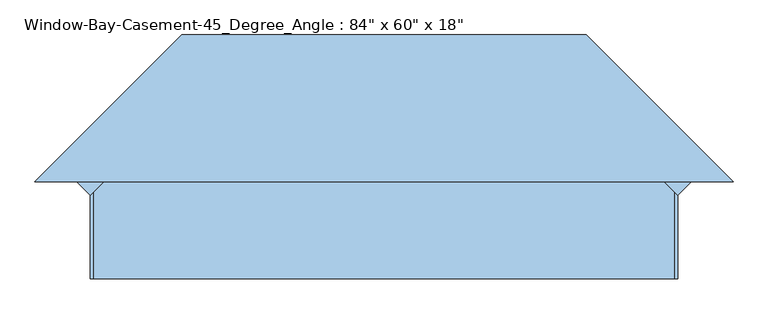
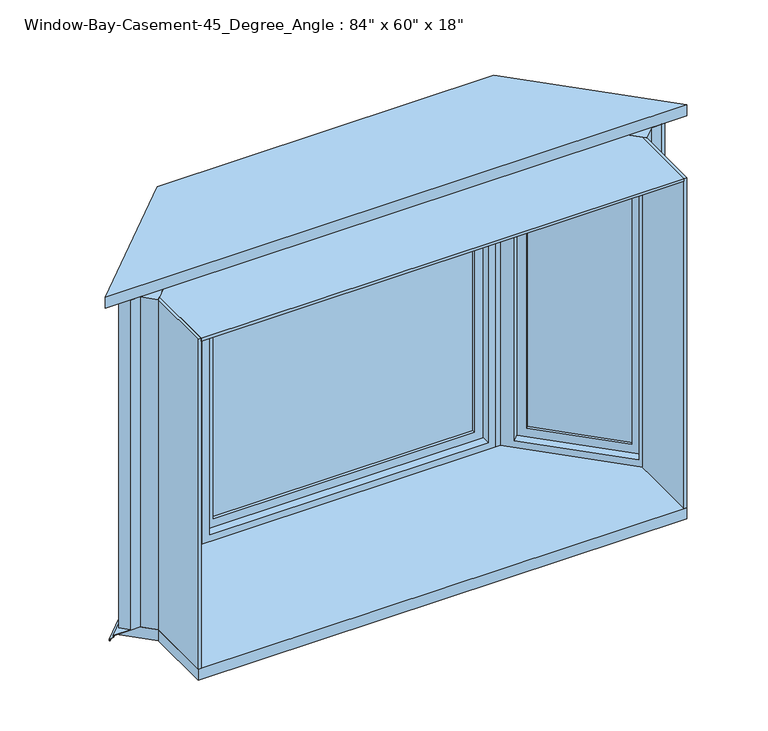
"""IFC4 building model written with IfcOpenShell, lengths in millimetres: window geometry."""

import ifcopenshell
import ifcopenshell.guid

model = None  # the IFC model being written
_history = None  # IfcOwnerHistory: only IFC2X3 demands one
_inside = {}  # id of a spatial element -> (the spatial element, [elements in it])
_under = {}  # id of a project, library or spatial element -> (it, [spatial elements below it])
_declared = {}  # id of a project -> (the project, [libraries it declares])
_typed = {}  # id of a type object -> (the type object, [elements of that type])
_made_of = {}  # id of a material, layer set ... -> (it, [elements and type objects made of it])


def new_model(schema):
    """Start an empty IFC model of exactly this schema.

    Asked for "IFC4X3", IfcOpenShell would pick the latest addendum, in which some entities
    have other attributes; the version numbers below select the first issue.
    IFC2X3 requires an IfcOwnerHistory on every rooted entity: one is made here for all.
    """
    global model, _history
    if schema == "IFC4X3":
        model = ifcopenshell.file(schema_version=(4, 3, 0, 0))
    else:
        model = ifcopenshell.file(schema=schema)
    _inside.clear()
    _under.clear()
    _declared.clear()
    _typed.clear()
    _made_of.clear()
    _history = None
    if model.schema == "IFC2X3":
        org = make("IfcOrganization", Name="unknown")
        user = make(
            "IfcPersonAndOrganization",
            ThePerson=make("IfcPerson", FamilyName="unknown"),
            TheOrganization=org,
        )
        app = make(
            "IfcApplication",
            ApplicationDeveloper=org,
            Version="unknown",
            ApplicationFullName="unknown",
            ApplicationIdentifier="unknown",
        )
        _history = make(
            "IfcOwnerHistory",
            OwningUser=user,
            OwningApplication=app,
            ChangeAction="ADDED",
            CreationDate=0,
        )
    return model


def make(cls, **values):
    """One entity of the class cls with the attributes given. An attribute that is None is left unset."""
    return model.create_entity(
        cls, **{name: value for name, value in values.items() if value is not None}
    )


def rooted(cls, **values):
    """An entity with a GlobalId (a new one), such as an element, a storey or a relation."""
    return make(cls, GlobalId=ifcopenshell.guid.new(), OwnerHistory=_history, **values)


def si_unit(unit_type, name, prefix=None):
    """IfcSIUnit, for example si_unit("LENGTHUNIT", "METRE", prefix="MILLI")."""
    return make("IfcSIUnit", UnitType=unit_type, Prefix=prefix, Name=name)


def assignment(units):
    """IfcUnitAssignment: the units of a project."""
    return None if units is None else make("IfcUnitAssignment", Units=units)


def point(xyz):
    """IfcCartesianPoint."""
    return None if xyz is None else make("IfcCartesianPoint", Coordinates=xyz)


def direction(xyz):
    """IfcDirection."""
    return None if xyz is None else make("IfcDirection", DirectionRatios=xyz)


def frame(location, z_axis=None, x_axis=None):
    """IfcAxis2Placement3D, a coordinate frame: its origin and axes. An axis left out is left unset."""
    return make(
        "IfcAxis2Placement3D",
        Location=point(location),
        Axis=direction(z_axis),
        RefDirection=direction(x_axis),
    )


def origin():
    """The frame at (0, 0, 0) with its axes left unset."""
    return frame((0.0, 0.0, 0.0))


def place(relative_to, where):
    """IfcLocalPlacement: puts the frame where relative to a parent placement (None: the world)."""
    return make(
        "IfcLocalPlacement", PlacementRelTo=relative_to, RelativePlacement=where
    )


def context(
    kind, dimensions, precision=None, world=None, true_north=None, identifier=None
):
    """IfcGeometricRepresentationContext, for example the 3D "Model" context."""
    return make(
        "IfcGeometricRepresentationContext",
        ContextIdentifier=identifier,
        ContextType=kind,
        CoordinateSpaceDimension=dimensions,
        Precision=precision,
        WorldCoordinateSystem=world,
        TrueNorth=true_north,
    )


def project(units=None, contexts=None):
    """IfcProject with its units and contexts."""
    return rooted(
        "IfcProject",
        Name="project",
        RepresentationContexts=contexts,
        UnitsInContext=assignment(units),
    )


def spatial(cls, under=None, at=None, **own):
    """A site, building, storey or space (cls), placed at a placement, below another one or the project."""
    s = rooted(cls, ObjectPlacement=at, **own)
    if under is not None:
        _under.setdefault(under.id(), (under, []))[1].append(s)
    return s


def polyline(points):
    """IfcPolyline through the points."""
    return make("IfcPolyline", Points=[point(p) for p in points])


def outline(outer, holes=None, kind="AREA"):
    """IfcArbitraryClosedProfileDef: a profile drawn as a closed curve; with holes, ...WithVoids."""
    if holes is None:
        return make("IfcArbitraryClosedProfileDef", ProfileType=kind, OuterCurve=outer)
    return make(
        "IfcArbitraryProfileDefWithVoids",
        ProfileType=kind,
        OuterCurve=outer,
        InnerCurves=holes,
    )


def extrude(swept, where, along, depth):
    """IfcExtrudedAreaSolid: the profile swept, set in the frame where, extruded along a direction by depth."""
    return make(
        "IfcExtrudedAreaSolid",
        SweptArea=swept,
        Position=where,
        ExtrudedDirection=direction(along),
        Depth=depth,
    )


def faces_of(points, faces, orient=None, outer=None):
    """IfcFace entities. A face is a list of loops; a loop is a list of indices into points, from 0.

    orient and outer hold one flag for each loop. By default every Orientation is true, the
    first loop of a face is its IfcFaceOuterBound and the others are IfcFaceBound.
    """
    made = []
    for i, loops in enumerate(faces):
        bounds = []
        for j, loop in enumerate(loops):
            is_outer = j == 0 if outer is None else outer[i][j]
            bounds.append(
                make(
                    "IfcFaceOuterBound" if is_outer else "IfcFaceBound",
                    Bound=make("IfcPolyLoop", Polygon=[points[k] for k in loop]),
                    Orientation=True if orient is None else orient[i][j],
                )
            )
        made.append(make("IfcFace", Bounds=bounds))
    return made


def faceted_brep(points, faces, orient=None, outer=None, voids=None):
    """IfcFacetedBrep: a solid bounded by flat faces; with voids (closed shells), ...WithVoids."""
    shared = [point(p) for p in points]
    hull = make("IfcClosedShell", CfsFaces=faces_of(shared, faces, orient, outer))
    if voids is None:
        return make("IfcFacetedBrep", Outer=hull)
    return make(
        "IfcFacetedBrepWithVoids",
        Outer=hull,
        Voids=[
            make(cls, CfsFaces=faces_of(shared, fs, o, b)) for cls, fs, o, b in voids
        ],
    )


def shape(context_of_items, identifier, shape_type, items):
    """IfcShapeRepresentation: the items that make up one representation, for example the "Body"."""
    return make(
        "IfcShapeRepresentation",
        ContextOfItems=context_of_items,
        RepresentationIdentifier=identifier,
        RepresentationType=shape_type,
        Items=items,
    )


def source(mapping_origin, context_of_items, identifier, shape_type, items):
    """IfcRepresentationMap: a shape defined once, which mapped items show again and again."""
    return make(
        "IfcRepresentationMap",
        MappingOrigin=mapping_origin,
        MappedRepresentation=shape(context_of_items, identifier, shape_type, items),
    )


def transform(
    local_origin,
    x_axis=None,
    y_axis=None,
    z_axis=None,
    scale=None,
    scale2=None,
    scale3=None,
    uniform=True,
):
    """IfcCartesianTransformationOperator3D, or its non-uniform kind. x_axis, y_axis, z_axis: its Axis1, 2, 3."""
    if uniform:
        return make(
            "IfcCartesianTransformationOperator3D",
            Axis1=direction(x_axis),
            Axis2=direction(y_axis),
            LocalOrigin=point(local_origin),
            Scale=scale,
            Axis3=direction(z_axis),
        )
    return make(
        "IfcCartesianTransformationOperator3DnonUniform",
        Axis1=direction(x_axis),
        Axis2=direction(y_axis),
        LocalOrigin=point(local_origin),
        Scale=scale,
        Axis3=direction(z_axis),
        Scale2=scale2,
        Scale3=scale3,
    )


def mapped(mapping_source, mapping_target):
    """IfcMappedItem: shows the shape of a source again, moved by a transform."""
    return make(
        "IfcMappedItem", MappingSource=mapping_source, MappingTarget=mapping_target
    )


def made_of(thing, what):
    """Note that an element or type object is made of a material, layer set ...; save() writes the relation."""
    if what is not None:
        _made_of.setdefault(what.id(), (what, []))[1].append(thing)
    return thing


def element(
    cls,
    number,
    at=None,
    inside=None,
    cuts=None,
    type_object=None,
    material=None,
    context=None,
    identifier="Body",
    shape_type=None,
    held_by="IfcProductDefinitionShape",
    body=None,
    shapes=None,
    **own,
):
    """One element of the class cls, such as IfcWall. Its Tag is "e" and its number.

    at: its placement. inside: the storey or other place that contains it. cuts: it is an
    opening in that element (IfcRelVoidsElement). A single representation is given by context,
    identifier, shape_type and body (its items); several are given by shapes. held_by: the class
    of the entity that holds the representations. save() writes the other relations.
    """
    e = rooted(cls, Tag="e%d" % number, ObjectPlacement=at, **own)
    if body is not None:
        shapes = [shape(context, identifier, shape_type, body)]
    if shapes is not None:
        e.Representation = make(held_by, Representations=shapes)
    if inside is not None:
        _inside.setdefault(inside.id(), (inside, []))[1].append(e)
    if cuts is not None:
        rooted(
            "IfcRelVoidsElement", RelatingBuildingElement=cuts, RelatedOpeningElement=e
        )
    if type_object is not None:
        _typed.setdefault(type_object.id(), (type_object, []))[1].append(e)
    return made_of(e, material)


def aggregate(whole, parts):
    """IfcRelAggregates: a whole, such as a stair, and the parts it consists of."""
    return rooted("IfcRelAggregates", RelatingObject=whole, RelatedObjects=parts)


def save(model, path):
    """Write the relations noted so far, then the file.

    IfcRelAggregates (storeys below a building ...), IfcRelContainedInSpatialStructure (elements
    in a storey), IfcRelDefinesByType, IfcRelAssociatesMaterial and IfcRelDeclares: one each for
    every whole, place, type object, material and project.
    """
    for whole, parts in _under.values():
        aggregate(whole, parts)
    for where, things in _inside.values():
        rooted(
            "IfcRelContainedInSpatialStructure",
            RelatedElements=things,
            RelatingStructure=where,
        )
    for kind, things in _typed.values():
        rooted("IfcRelDefinesByType", RelatedObjects=things, RelatingType=kind)
    for what, things in _made_of.values():
        rooted("IfcRelAssociatesMaterial", RelatedObjects=things, RelatingMaterial=what)
    for by, libraries in _declared.values():
        rooted("IfcRelDeclares", RelatingContext=by, RelatedDefinitions=libraries)
    model.write(path)


def window_84e65bd0(model_context):
    return source(origin(), model_context, "Body", "SolidModel", [
        extrude(outline(polyline([(1066.8, 225.6039087), (1062.3098719, 221.1137806), (771.5637138, 511.8599388), (776.0538418, 516.3500668), (1066.8, 225.6039087)])), frame((0.0, 0.0, 730.25), z_axis=(0.0, 0.0, 1.0), x_axis=(1.0, 0.0, 0.0)), (0.0, 0.0, 1.0), 1384.3),
        extrude(outline(polyline([(1057.8197439, 216.6236525), (1053.3296158, 212.1335245), (762.5834576, 502.8796827), (767.0735857, 507.3698107), (1057.8197439, 216.6236525)])), frame((0.0, 0.0, 730.25), z_axis=(0.0, 0.0, 1.0), x_axis=(1.0, 0.0, 0.0)), (0.0, 0.0, 1.0), 1384.3),
        extrude(outline(polyline([(1441.45, 57.15), (1441.45, -468.3271601), (-57.15, -468.3271601), (-57.15, 57.15), (1441.45, 57.15)]), holes=[polyline([(1384.3, -411.1771601), (1384.3, 0.0), (0.0, 0.0), (0.0, -411.1771601), (1384.3, -411.1771601)])]), frame((1044.3493597, 203.1532684, 730.25), z_axis=(0.7071067811865468, 0.7071067811865483, 0.0), x_axis=(0.0, 0.0, 1.0)), (0.0, 0.0, 1.0), 44.45),
        faceted_brep([(661.8085913, 531.8125, 2184.4), (1066.8, 126.8210913, 2184.4), (1116.1914087, 176.2125, 2184.4), (1161.0926893, 176.2125, 2184.4), (703.8926893, 633.4125, 2184.4), (1084.7605122, 162.7421158, 2171.7), (713.192049, 534.3105791, 2171.7), (758.0933296, 579.2118597, 2171.7), (1129.6617928, 207.6433964, 2171.7), (1044.3493597, 149.2717316, 2152.65), (699.7216648, 493.8994265, 2152.65), (726.6624332, 520.8401949, 2152.65), (1071.2901281, 176.2125, 2152.65), (713.192049, 534.3105791, 673.1), (758.0933296, 579.2118597, 673.1), (699.7216648, 493.8994265, 692.15), (726.6624332, 520.8401949, 692.15), (703.8926893, 633.4125, 660.4), (1161.0926893, 176.2125, 660.4), (1116.1914087, 176.2125, 660.4), (1066.8, 126.8210913, 660.4), (661.8085913, 531.8125, 660.4), (1084.7605122, 162.7421158, 673.1), (1129.6617928, 207.6433964, 673.1), (1044.3493597, 149.2717316, 692.15), (1071.2901281, 176.2125, 692.15)], [[[0, 1, 2, 3, 4]], [[5, 6, 7, 8]], [[9, 10, 11, 12]], [[6, 13, 14, 7]], [[10, 15, 16, 11]], [[17, 18, 19, 20, 21]], [[13, 22, 23, 14]], [[15, 24, 25, 16]], [[20, 19, 2, 1]], [[3, 18, 17, 4], [7, 14, 23, 8]], [[8, 23, 22, 5]], [[5, 22, 13, 6], [11, 16, 25, 12]], [[12, 25, 24, 9]], [[1, 0, 21, 20], [9, 24, 15, 10]], [[4, 17, 21, 0]], [[2, 19, 18, 3]]]),
        extrude(outline(polyline([(-1066.8, 225.6039087), (-776.0538418, 516.3500668), (-771.5637138, 511.8599388), (-1062.3098719, 221.1137806), (-1066.8, 225.6039087)])), frame((0.0, 0.0, 730.25), z_axis=(0.0, 0.0, 1.0), x_axis=(1.0, 0.0, 0.0)), (0.0, 0.0, 1.0), 1384.3),
        extrude(outline(polyline([(-1057.8197439, 216.6236525), (-767.0735857, 507.3698107), (-762.5834576, 502.8796827), (-1053.3296158, 212.1335245), (-1057.8197439, 216.6236525)])), frame((0.0, 0.0, 730.25), z_axis=(0.0, 0.0, 1.0), x_axis=(1.0, 0.0, 0.0)), (0.0, 0.0, 1.0), 1384.3),
        extrude(outline(polyline([(1441.45, -57.15), (-57.15, -57.15), (-57.15, 468.3271601), (1441.45, 468.3271601), (1441.45, -57.15)]), holes=[polyline([(1384.3, 411.1771601), (0.0, 411.1771601), (0.0, 0.0), (1384.3, 0.0), (1384.3, 411.1771601)])]), frame((-1044.3493597, 203.1532684, 730.25), z_axis=(-0.7071067811865468, 0.7071067811865483, 0.0), x_axis=(0.0, 0.0, 1.0)), (0.0, 0.0, 1.0), 44.45),
        faceted_brep([(-661.8085913, 531.8125, 2184.4), (-703.8926893, 633.4125, 2184.4), (-1161.0926893, 176.2125, 2184.4), (-1116.1914087, 176.2125, 2184.4), (-1066.8, 126.8210913, 2184.4), (-1084.7605122, 162.7421158, 2171.7), (-1129.6617928, 207.6433964, 2171.7), (-758.0933296, 579.2118597, 2171.7), (-713.192049, 534.3105791, 2171.7), (-1044.3493597, 149.2717316, 2152.65), (-1071.2901281, 176.2125, 2152.65), (-726.6624332, 520.8401949, 2152.65), (-699.7216648, 493.8994265, 2152.65), (-758.0933296, 579.2118597, 673.1), (-713.192049, 534.3105791, 673.1), (-726.6624332, 520.8401949, 692.15), (-699.7216648, 493.8994265, 692.15), (-703.8926893, 633.4125, 660.4), (-661.8085913, 531.8125, 660.4), (-1066.8, 126.8210913, 660.4), (-1116.1914087, 176.2125, 660.4), (-1161.0926893, 176.2125, 660.4), (-1129.6617928, 207.6433964, 673.1), (-1084.7605122, 162.7421158, 673.1), (-1071.2901281, 176.2125, 692.15), (-1044.3493597, 149.2717316, 692.15)], [[[0, 1, 2, 3, 4]], [[5, 6, 7, 8]], [[9, 10, 11, 12]], [[8, 7, 13, 14]], [[12, 11, 15, 16]], [[17, 18, 19, 20, 21]], [[14, 13, 22, 23]], [[16, 15, 24, 25]], [[19, 4, 3, 20]], [[2, 1, 17, 21], [7, 6, 22, 13]], [[6, 5, 23, 22]], [[5, 8, 14, 23], [11, 10, 24, 15]], [[10, 9, 25, 24]], [[4, 19, 18, 0], [9, 12, 16, 25]], [[1, 0, 18, 17]], [[3, 2, 21, 20]]]),
        faceted_brep([(-724.9347382, 684.2125, 660.4), (-724.9347382, 684.2125, 653.0697935), (724.9347382, 684.2125, 653.0697935), (724.9347382, 684.2125, 660.4), (-703.8926893, 633.4125, 663.1486341), (-703.8926893, 633.4125, 660.4), (703.8926893, 633.4125, 660.4), (703.8926893, 633.4125, 663.1486341), (-725.5133946, 685.6095, 654.4483503), (-725.5133946, 685.6095, 663.1486341), (725.5133946, 685.6095, 663.1486341), (725.5133946, 685.6095, 654.4483503), (730.7739068, 698.3095, 652.2089977), (-730.7739068, 698.3095, 652.2089977), (730.7739068, 698.3095, 643.2668038), (-730.7739068, 698.3095, 643.2668038), (-729.132627, 694.3471, 644.7270038), (-729.132627, 694.3471, 643.2668038), (729.132627, 694.3471, 643.2668038), (729.132627, 694.3471, 644.7270038), (-730.1110823, 696.7093, 650.8662705), (-730.1110823, 696.7093, 644.7270038), (730.1110823, 696.7093, 644.7270038), (730.1110823, 696.7093, 650.8662705), (-1232.9347382, 176.2125, 660.4), (-1232.9347382, 176.2125, 653.0697935), (1232.9347382, 176.2125, 660.4), (1161.0926893, 176.2125, 660.4), (-1161.0926893, 176.2125, 660.4), (-1161.0926893, 176.2125, 663.1486341), (1161.0926893, 176.2125, 663.1486341), (1234.9103945, 176.2125, 663.1486341), (-1234.9103945, 176.2125, 663.1486341), (-1234.9103945, 176.2125, 654.4483503), (-1252.8709068, 176.2125, 652.2089977), (-1252.8709068, 176.2125, 643.2668038), (1252.8709068, 176.2125, 643.2668038), (1247.2672271, 176.2125, 643.2668038), (-1247.2672271, 176.2125, 643.2668038), (-1247.2672271, 176.2125, 644.7270038), (1247.2672271, 176.2125, 644.7270038), (1250.6078823, 176.2125, 644.7270038), (-1250.6078823, 176.2125, 644.7270038), (-1250.6078823, 176.2125, 650.8662705), (1232.9347382, 176.2125, 653.0697935), (1234.9103945, 176.2125, 654.4483503), (1252.8709068, 176.2125, 652.2089977), (1250.6078823, 176.2125, 650.8662705)], [[[0, 1, 2, 3]], [[4, 5, 6, 7]], [[8, 9, 10, 11]], [[8, 11, 12, 13]], [[13, 12, 14, 15]], [[16, 17, 18, 19]], [[20, 21, 22, 23]], [[2, 1, 20, 23]], [[1, 0, 24, 25]], [[0, 3, 26, 27, 6, 5, 28, 24]], [[5, 4, 29, 28]], [[4, 7, 30, 31, 10, 9, 32, 29]], [[9, 8, 33, 32]], [[8, 13, 34, 33]], [[13, 15, 35, 34]], [[15, 14, 36, 37, 18, 17, 38, 35]], [[17, 16, 39, 38]], [[16, 19, 40, 41, 22, 21, 42, 39]], [[21, 20, 43, 42]], [[20, 1, 25, 43]], [[3, 2, 44, 26]], [[7, 6, 27, 30]], [[11, 10, 31, 45]], [[12, 11, 45, 46]], [[14, 12, 46, 36]], [[19, 18, 37, 40]], [[23, 22, 41, 47]], [[2, 23, 47, 44]], [[25, 24, 28, 29, 32, 33, 34, 35, 38, 39, 42, 43]], [[27, 26, 44, 47, 41, 40, 37, 36, 46, 45, 31, 30]]]),
        extrude(outline(polyline([(-1138.642049, 198.6631403), (-1161.0926893, 176.2125), (-1192.5235857, 207.6433964), (-1170.0729454, 230.0940367), (-1138.642049, 198.6631403)])), frame((0.0, 0.0, 663.1486341), z_axis=(0.0, 0.0, 1.0), x_axis=(1.0, 0.0, 0.0)), (0.0, 0.0, 1.0), 1521.2513659),
        extrude(outline(polyline([(1138.642049, 198.6631403), (1170.0729454, 230.0940367), (1192.5235857, 207.6433964), (1161.0926893, 176.2125), (1138.642049, 198.6631403)])), frame((0.0, 0.0, 663.1486341), z_axis=(0.0, 0.0, 1.0), x_axis=(1.0, 0.0, 0.0)), (0.0, 0.0, 1.0), 1521.2513659),
        extrude(outline(polyline([(-661.8085913, 531.8125), (661.8085913, 531.8125), (1054.1, 139.5210913), (1054.1, -176.2125), (-1054.1, -176.2125), (-1054.1, 139.5210913), (-661.8085913, 531.8125)])), frame((0.0, 0.0, 2171.7), z_axis=(0.0, 0.0, 1.0), x_axis=(1.0, 0.0, 0.0)), (0.0, 0.0, 1.0), 12.7),
        extrude(outline(polyline([(-1066.8, -176.2125), (-1066.8, 126.8210913), (-1054.1, 139.5210913), (-1054.1, -176.2125), (-1066.8, -176.2125)])), frame((0.0, 0.0, 660.4), z_axis=(0.0, 0.0, 1.0), x_axis=(1.0, 0.0, 0.0)), (0.0, 0.0, 1.0), 1524.0),
        extrude(outline(polyline([(1066.8, -176.2125), (1054.1, -176.2125), (1054.1, 139.5210913), (1066.8, 126.8210913), (1066.8, -176.2125)])), frame((0.0, 0.0, 660.4), z_axis=(0.0, 0.0, 1.0), x_axis=(1.0, 0.0, 0.0)), (0.0, 0.0, 1.0), 1524.0),
        extrude(outline(polyline([(2171.7, -627.2414087), (673.1, -627.2414087), (673.1, 627.2414087), (2171.7, 627.2414087), (2171.7, -627.2414087)]), holes=[polyline([(2114.55, 570.0914087), (730.25, 570.0914087), (730.25, -570.0914087), (2114.55, -570.0914087), (2114.55, 570.0914087)])]), frame((0.0, 569.9125, 0.0), z_axis=(0.0, 1.0, 0.0), x_axis=(0.0, 0.0, 1.0)), (0.0, 0.0, 1.0), 44.45),
        extrude(outline(polyline([(1066.8, -176.2125), (-1066.8, -176.2125), (-1066.8, 126.8210913), (-1174.5630735, 234.5841648), (-724.9347382, 684.2125), (724.9347382, 684.2125), (1174.5630735, 234.5841648), (1066.8, 126.8210913), (1066.8, -176.2125)])), frame((0.0, 0.0, 609.6), z_axis=(0.0, 0.0, 1.0), x_axis=(1.0, 0.0, 0.0)), (0.0, 0.0, 1.0), 50.8),
        extrude(outline(polyline([(570.0914087, 601.6625), (570.0914087, 595.3125), (-570.0914087, 595.3125), (-570.0914087, 601.6625), (570.0914087, 601.6625)])), frame((0.0, 0.0, 730.25), z_axis=(0.0, 0.0, 1.0), x_axis=(1.0, 0.0, 0.0)), (0.0, 0.0, 1.0), 1384.3),
        extrude(outline(polyline([(570.0914087, 588.9625), (570.0914087, 582.6125), (-570.0914087, 582.6125), (-570.0914087, 588.9625), (570.0914087, 588.9625)])), frame((0.0, 0.0, 730.25), z_axis=(0.0, 0.0, 1.0), x_axis=(1.0, 0.0, 0.0)), (0.0, 0.0, 1.0), 1384.3),
        faceted_brep([(627.2414087, 569.9125, 673.1), (627.2414087, 633.4125, 673.1), (-627.2414087, 633.4125, 673.1), (-627.2414087, 569.9125, 673.1), (608.1914087, 531.8125, 692.15), (608.1914087, 569.9125, 692.15), (-608.1914087, 569.9125, 692.15), (-608.1914087, 531.8125, 692.15), (639.9414087, 633.4125, 660.4), (639.9414087, 531.8125, 660.4), (-639.9414087, 531.8125, 660.4), (-639.9414087, 633.4125, 660.4), (-627.2414087, 633.4125, 2171.7), (-627.2414087, 569.9125, 2171.7), (-608.1914087, 569.9125, 2152.65), (-608.1914087, 531.8125, 2152.65), (-639.9414087, 531.8125, 2184.4), (-639.9414087, 633.4125, 2184.4), (627.2414087, 633.4125, 2171.7), (627.2414087, 569.9125, 2171.7), (608.1914087, 569.9125, 2152.65), (608.1914087, 531.8125, 2152.65), (639.9414087, 531.8125, 2184.4), (639.9414087, 633.4125, 2184.4)], [[[0, 1, 2, 3]], [[4, 5, 6, 7]], [[8, 9, 10, 11]], [[3, 2, 12, 13]], [[7, 6, 14, 15]], [[11, 10, 16, 17]], [[13, 12, 18, 19]], [[15, 14, 20, 21]], [[17, 16, 22, 23]], [[11, 17, 23, 8], [1, 18, 12, 2]], [[19, 18, 1, 0]], [[3, 13, 19, 0], [5, 20, 14, 6]], [[21, 20, 5, 4]], [[9, 22, 16, 10], [7, 15, 21, 4]], [[23, 22, 9, 8]]]),
        extrude(outline(polyline([(-639.9414087, 633.4125), (-639.9414087, 531.8125), (-661.8085913, 531.8125), (-703.8926893, 633.4125), (-639.9414087, 633.4125)])), frame((0.0, 0.0, 660.4), z_axis=(0.0, 0.0, 1.0), x_axis=(1.0, 0.0, 0.0)), (0.0, 0.0, 1.0), 1524.0),
        extrude(outline(polyline([(703.8926893, 633.4125), (661.8085913, 531.8125), (639.9414087, 531.8125), (639.9414087, 633.4125), (703.8926893, 633.4125)])), frame((0.0, 0.0, 660.4), z_axis=(0.0, 0.0, 1.0), x_axis=(1.0, 0.0, 0.0)), (0.0, 0.0, 1.0), 1524.0),
        extrude(outline(polyline([(735.4557627, 709.6125), (1268.8557627, 176.2125), (-1268.8557627, 176.2125), (-735.4557627, 709.6125), (735.4557627, 709.6125)])), frame((0.0, 0.0, 2184.4), z_axis=(0.0, 0.0, 1.0), x_axis=(1.0, 0.0, 0.0)), (0.0, 0.0, 1.0), 50.8),
    ])


if __name__ == "__main__":
    model = new_model("IFC4")
    model_context = context("Model", 3, world=origin())
    ifc_project = project(units=[si_unit("LENGTHUNIT", "METRE", prefix="MILLI")], contexts=[model_context])
    site = spatial("IfcSite", under=ifc_project)
    building = spatial("IfcBuilding", under=site)
    placement = place(None, origin())
    window_shape = window_84e65bd0(model_context)
    element("IfcWindow", 1, ObjectType="Window-Bay-Casement-45_Degree_Angle : 84\" x 60\" x 18\"", at=placement, inside=building, context=model_context, shape_type="MappedRepresentation", body=[
        mapped(window_shape, transform((0.0, 0.0, 0.0), x_axis=(1.0, 0.0, 0.0), y_axis=(0.0, 1.0, 0.0), z_axis=(0.0, 0.0, 1.0))),
    ])
    save(model, "model.ifc")

# Revit data of these elements
# Type "Window-Bay-Casement-45_Degree_Angle : 84\" x 60\" x 18\""
#   Type Mark = "27"
#   Fire Rating = "0.5h"
#   Assembly Code = "B2020100"
#   Analytic Construction = "Double glazing - domestic"
#   Width of Middle Sash = 4' - 2.38909"
#   Width = 7' - 0"
#   Visual Light Transmittance = 0.81
#   Thermal Resistance (R) = 1.8146 (h·ft²·°F)/BTU
#   Solar Heat Gain Coefficient = 0.76
#   Rough Width = 7' - 0 1/2"
#   Rough Height = 5' - 0 1/2"
#   Length 4 = 0' - 1.13909"
#   Length 3 = 0' - 0.51777"
#   Length 2 = 4' - 7.42462"
#   Length 1 = 1' - 2.80546"
#   Wall Thickness [instance default] = 0' - 6"
#   Trim Width = 7' - 5.03553"
#   Trim Height = 5' - 0"
#   Height 1 = 5' - 2"
#   Height = 5' - 0"
#   Heat Transfer Coefficient (U) = 0.5511 BTU/(h·ft²·°F)
#   Depth = 1' - 6"
#   Default Sill Height = 2' - 0"
#   Angle 1 = 22.5000°
#   Angle = 45.0000°
#   Center Muntin Visibility = yes
#   Side Muntin Visibility = yes
#   Interior Trim Visibility [instance default] = yes
#   Exterior Trim Visibility [instance default] = yes
#   Center Muntin Pattern = Muntin Pattern_2x2 : Muntin Pattern_2x2
#   Side Muntin Pattern = Muntin Pattern_2x2 : Muntin Pattern_2x2
#   Interior Trim Material = Wood - Stained
#   Exterior Trim Material = Clad - White
#   Exterior Trim = element 422174
#   Interior Trim = Trim-Window-Interior-Flat : Picture Frame
#   Interior Frame Material = Wood - Stained
#   Glass Panel Material = Glass
#   Exterior Frame Material = Clad - White
#   Wall Closure = (empty or 0)
# Element 1 (IfcWindow, "Window-Bay-Casement-45_Degree_Angle : 84\" x 60\" x 18\"")
#   Wall Thickness = 1' - 1 7/8"
#   Materials on its faces: "Wood - Stained", "Clad - White", "Glass"
# Materials
#   "Wood - Stained": class "Wood", colour RGB 224 178 126, transparency 0, Cost = 0
#   "Clad - White": class "Wood", colour RGB 242 242 238, transparency 0, Cost = 0
#   "Glass": class "Glass", colour RGB 0 128 192, transparency 0.75, Description = "Soda Lime Glass", Cost = 0
